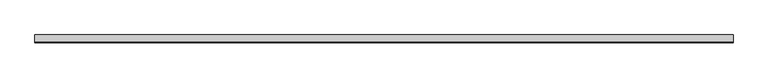
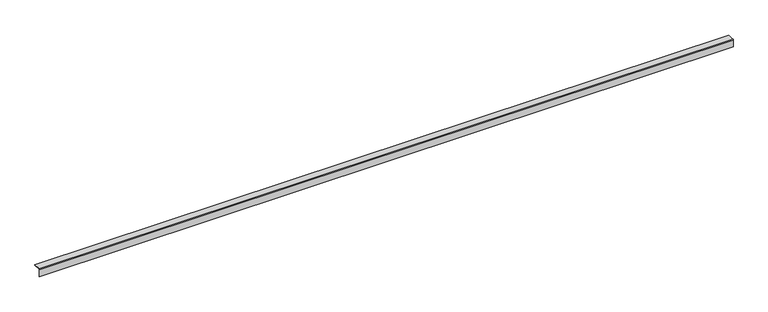
"""IFC4 building model written with IfcOpenShell, lengths in millimetres: proxy geometry, Metal profile007 2198 : Metal profile007 2198."""

from ifc_helpers import new_model, si_unit, point, frame, frame_2d, origin, place, context, project, spatial, polyline, circle_curve, trimmed, segment, composite_curve, outline, extrude, source, transform, mapped, element, save


def generic_models_183138f6(model_context):
    return source(origin(), model_context, "Body", "SweptSolid", [
        extrude(outline(composite_curve([segment(polyline([(9598.7832673, 37512.0598437), (9577.6300834, 37512.0598437), (9577.6300834, 37490.9066598), (9576.3500834, 37490.9066598), (9576.3500834, 37511.8095695)]), True, "CONTINUOUS"), segment(trimmed(circle_curve(frame_2d((9576.9900834, 37512.6998437)), 1.0964434), [point((9576.3500834, 37511.8095695))], [point((9577.8803576, 37513.3398437))], False, "CARTESIAN"), True, "CONTINUOUS"), segment(polyline([(9577.8803576, 37513.3398437), (9598.7832673, 37513.3398437), (9598.7832673, 37512.0598437)]), True, "CONTINUOUS")], self_intersect=False)), frame((3694.2883192, 0.0, 0.0), z_axis=(1.0, 0.0, 0.0), x_axis=(0.0, 1.0, 0.0)), (0.0, 0.0, 1.0), 2000.0),
    ])


if __name__ == "__main__":
    model = new_model("IFC4")
    model_context = context("Model", 3, world=origin())
    ifc_project = project(units=[si_unit("LENGTHUNIT", "METRE", prefix="MILLI")], contexts=[model_context])
    site = spatial("IfcSite", under=ifc_project)
    building = spatial("IfcBuilding", under=site)
    placement = place(None, origin())
    generic_models_shape = generic_models_183138f6(model_context)
    element("IfcBuildingElementProxy", 1, Name="Metal profile007 2198 : Metal profile007 2198", ObjectType="Metal profile007 2198 : Metal profile007 2198", at=placement, inside=building, context=model_context, shape_type="MappedRepresentation", body=[
        mapped(generic_models_shape, transform((0.0, 0.0, 0.0), x_axis=(1.0, 0.0, 0.0), y_axis=(0.0, 1.0, 0.0), z_axis=(0.0, 0.0, 1.0))),
    ])
    save(model, "model.ifc")

# Revit data of these elements
# Type "Metal profile007 2198 : Metal profile007 2198"
#   NameOverride = "Metal profile007"
# Element 1 (IfcBuildingElementProxy, "Metal profile007 2198 : Metal profile007 2198")
#   Materials on its faces: "CORNER BEAD"
# Materials
#   "CORNER BEAD": class "Unassigned", colour RGB 255 241 0, transparency 0
